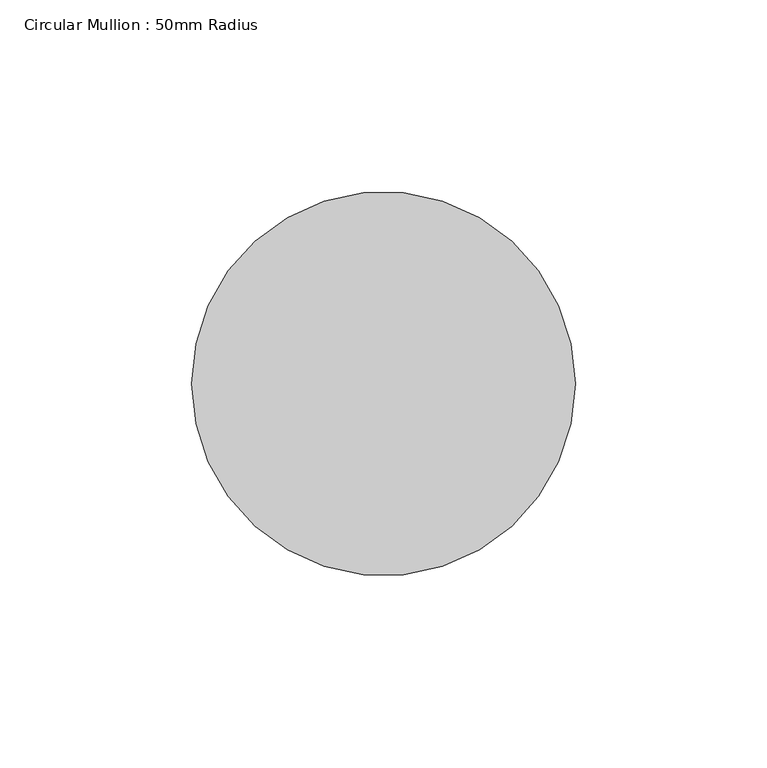
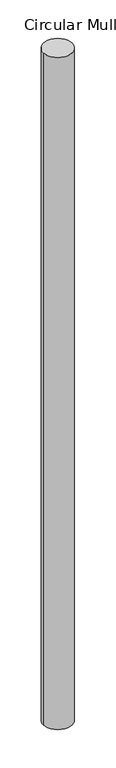
"""IFC4 building model written with IfcOpenShell, lengths in millimetres: member geometry, Circular Mullion : 50mm Radius."""

from ifc_helpers import new_model, si_unit, point, frame, frame_2d, origin, place, context, project, spatial, circle_curve, trimmed, segment, composite_curve, outline, extrude, source, transform, mapped, element, save


def circular_mullion_50mm_radius_04dfe012(model_context):
    return source(origin(), model_context, "Body", "SweptSolid", [
        extrude(outline(composite_curve([segment(trimmed(circle_curve(frame_2d((-50.0, 0.0)), 50.0), [point((0.0, 0.0))], [point((-100.0, 0.0))], False, "CARTESIAN"), True, "CONTINUOUS"), segment(trimmed(circle_curve(frame_2d((-50.0, 0.0)), 50.0), [point((-100.0, 0.0))], [point((0.0, 0.0))], False, "CARTESIAN"), True, "CONTINUOUS")], self_intersect=False)), frame((0.0, 0.0, -2447.116324), z_axis=(0.0, 0.0, 1.0), x_axis=(1.0, 0.0, 0.0)), (0.0, 0.0, 1.0), 2447.116324),
    ])


if __name__ == "__main__":
    model = new_model("IFC4")
    model_context = context("Model", 3, world=origin())
    ifc_project = project(units=[si_unit("LENGTHUNIT", "METRE", prefix="MILLI")], contexts=[model_context])
    site = spatial("IfcSite", under=ifc_project)
    building = spatial("IfcBuilding", under=site)
    placement = place(None, origin())
    circular_mullion_50mm_radius_shape = circular_mullion_50mm_radius_04dfe012(model_context)
    element("IfcMember", 1, ObjectType="Circular Mullion : 50mm Radius", at=placement, inside=building, context=model_context, shape_type="MappedRepresentation", body=[
        mapped(circular_mullion_50mm_radius_shape, transform((0.0, 0.0, 0.0), x_axis=(1.0, 0.0, 0.0), y_axis=(0.0, 1.0, 0.0), z_axis=(0.0, 0.0, 1.0))),
    ])
    save(model, "model.ifc")

# Revit data of these elements
# Type "Circular Mullion : 50mm Radius"
#   built-in parameter 1007350 = 0.164042 (stored number, unit not read)
# Element 1 (IfcMember, "Circular Mullion : 50mm Radius")
#   Materials on its faces: "Aluminium"
# Materials
#   "Aluminium": class "Metal", colour RGB 247 247 247, transparency 0, Description = "Aluminium 6061", Cost = 0
